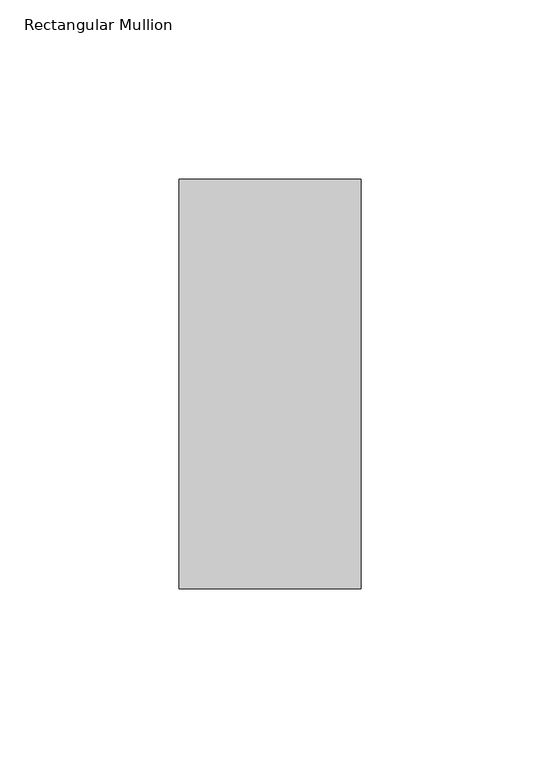
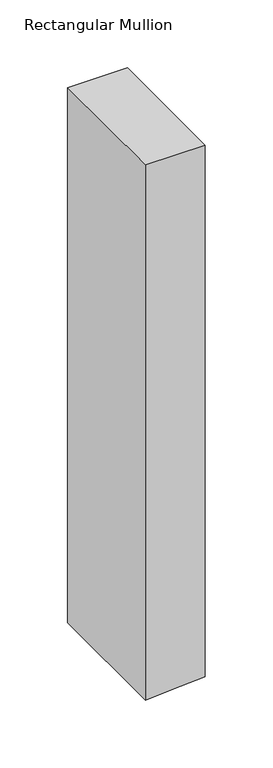
"""IFC4 building model written with IfcOpenShell, lengths in millimetres: member geometry, Rectangular Mullion : KAWNEER TRIFAB VERSAGLAZE 451T - CLEAR ANODIZED ALUM. - BACK GLAZED."""

from ifc_helpers import new_model, si_unit, frame, origin, place, context, project, spatial, polyline, outline, extrude, source, transform, mapped, element, save


def rectangular_mullion_ea686153(model_context):
    return source(origin(), model_context, "Body", "SweptSolid", [
        extrude(outline(polyline([(0.0, 25.4), (0.0, -25.4), (-481.0622061, -25.4), (-479.6727571, -3.1688169), (-477.8872061, 25.4), (0.0, 25.4)])), frame((0.0, -57.15, 0.0), z_axis=(0.0, 1.0, 0.0), x_axis=(0.0, 0.0, 1.0)), (0.0, 0.0, 1.0), 114.3),
    ])


if __name__ == "__main__":
    model = new_model("IFC4")
    model_context = context("Model", 3, world=origin())
    ifc_project = project(units=[si_unit("LENGTHUNIT", "METRE", prefix="MILLI")], contexts=[model_context])
    site = spatial("IfcSite", under=ifc_project)
    building = spatial("IfcBuilding", under=site)
    placement = place(None, origin())
    rectangular_mullion_shape = rectangular_mullion_ea686153(model_context)
    element("IfcMember", 1, ObjectType="Rectangular Mullion : KAWNEER TRIFAB VERSAGLAZE 451T - CLEAR ANODIZED ALUM. - BACK GLAZED", at=placement, inside=building, context=model_context, shape_type="MappedRepresentation", body=[
        mapped(rectangular_mullion_shape, transform((0.0, 0.0, 0.0), x_axis=(1.0, 0.0, 0.0), y_axis=(0.0, 1.0, 0.0), z_axis=(0.0, 0.0, 1.0))),
    ])
    save(model, "model.ifc")

# Revit data of these elements
# Type "Rectangular Mullion : KAWNEER TRIFAB VERSAGLAZE 451T - CLEAR ANODIZED ALUM. - BACK GLAZED"
#   built-in parameter 1007304 = 0.375 (stored number, unit not read)
#   built-in parameter 1007301 = 0.0833333 (stored number, unit not read)
#   built-in parameter 1007300 = 0.0833333 (stored number, unit not read)
# Element 1 (IfcMember, "Rectangular Mullion : KAWNEER TRIFAB VERSAGLAZE 451T - CLEAR ANODIZED ALUM. - BACK GLAZED")
#   Materials on its faces: "KAWNEER TRIFAB VERSAGLAZE 451T - CLEAR ANODIZED ALUM. - BACK GLAZED"
# Materials
#   "KAWNEER TRIFAB VERSAGLAZE 451T - CLEAR ANODIZED ALUM. - BACK GLAZED": class "Metal", colour RGB 244 244 244, transparency 0, Description = "Aluminum 6061", Cost = 0
